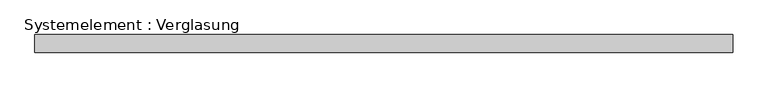
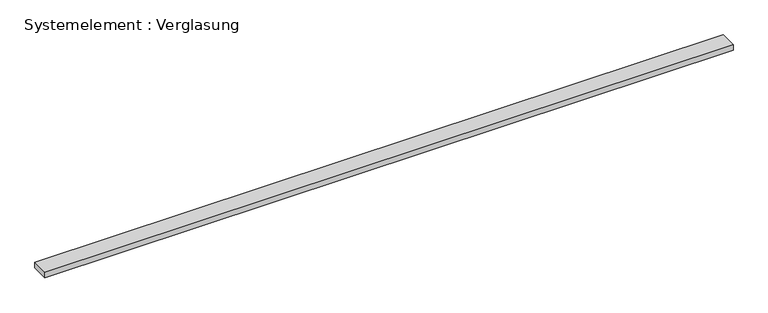
"""IFC4 building model written with IfcOpenShell, lengths in millimetres: plate geometry, Systemelement : Verglasung."""

from ifc_helpers import new_model, si_unit, origin, origin_with_axes, place, context, project, spatial, polyline, outline, extrude, source, transform, mapped, element, save


def systemelement_verglasung_dd9543b1(model_context):
    return source(origin(), model_context, "Body", "SweptSolid", [
        extrude(outline(polyline([(595.0, -15.0), (-595.0, -15.0), (-595.0, 15.0), (595.0, 15.0), (595.0, -15.0)])), origin_with_axes(), (0.0, 0.0, 1.0), 10.0),
    ])


if __name__ == "__main__":
    model = new_model("IFC4")
    model_context = context("Model", 3, world=origin())
    ifc_project = project(units=[si_unit("LENGTHUNIT", "METRE", prefix="MILLI")], contexts=[model_context])
    site = spatial("IfcSite", under=ifc_project)
    building = spatial("IfcBuilding", under=site)
    placement = place(None, origin())
    systemelement_verglasung_shape = systemelement_verglasung_dd9543b1(model_context)
    element("IfcPlate", 1, ObjectType="Systemelement : Verglasung", at=placement, inside=building, context=model_context, shape_type="MappedRepresentation", body=[
        mapped(systemelement_verglasung_shape, transform((0.0, 0.0, 0.0), x_axis=(1.0, 0.0, 0.0), y_axis=(0.0, 1.0, 0.0), z_axis=(0.0, 0.0, 1.0))),
    ])
    save(model, "model.ifc")

# Revit data of these elements
# Type "Systemelement : Verglasung"
#   Construction Type Id = "GSP4R"
#   Analytic Construction = "1/8 Zoll Pilkington-Verglasung einfach"
#   Visual Light Transmittance = 0.9
#   Solar Heat Gain Coefficient = 0.86
#   Heat Transfer Coefficient (U) = 6.7069 W/(m²·K)
# Element 1 (IfcPlate, "Systemelement : Verglasung")
#   Materials on its faces: "Glas"
# Materials
#   "Glas": class "Glas", colour RGB 0 0 255, transparency 0.75, Comments = "Render-Darstellung nicht aktualisiert ", Cost = 0
